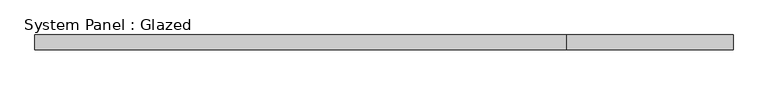
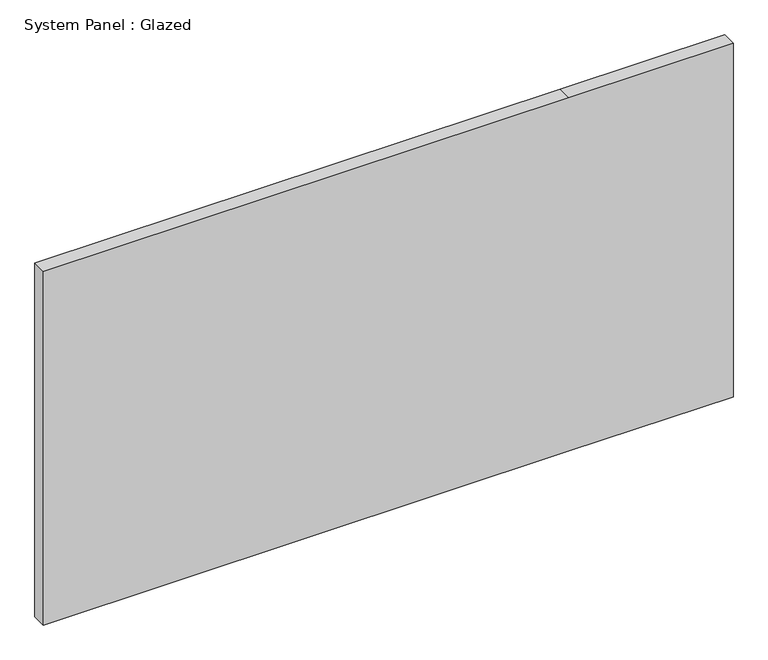
"""IFC4 building model written with IfcOpenShell, lengths in millimetres: plate geometry, System Panel : Glazed."""

import ifcopenshell
import ifcopenshell.guid

model = None  # the IFC model being written
_history = None  # IfcOwnerHistory: only IFC2X3 demands one
_inside = {}  # id of a spatial element -> (the spatial element, [elements in it])
_under = {}  # id of a project, library or spatial element -> (it, [spatial elements below it])
_declared = {}  # id of a project -> (the project, [libraries it declares])
_typed = {}  # id of a type object -> (the type object, [elements of that type])
_made_of = {}  # id of a material, layer set ... -> (it, [elements and type objects made of it])


def new_model(schema):
    """Start an empty IFC model of exactly this schema.

    Asked for "IFC4X3", IfcOpenShell would pick the latest addendum, in which some entities
    have other attributes; the version numbers below select the first issue.
    IFC2X3 requires an IfcOwnerHistory on every rooted entity: one is made here for all.
    """
    global model, _history
    if schema == "IFC4X3":
        model = ifcopenshell.file(schema_version=(4, 3, 0, 0))
    else:
        model = ifcopenshell.file(schema=schema)
    _inside.clear()
    _under.clear()
    _declared.clear()
    _typed.clear()
    _made_of.clear()
    _history = None
    if model.schema == "IFC2X3":
        org = make("IfcOrganization", Name="unknown")
        user = make(
            "IfcPersonAndOrganization",
            ThePerson=make("IfcPerson", FamilyName="unknown"),
            TheOrganization=org,
        )
        app = make(
            "IfcApplication",
            ApplicationDeveloper=org,
            Version="unknown",
            ApplicationFullName="unknown",
            ApplicationIdentifier="unknown",
        )
        _history = make(
            "IfcOwnerHistory",
            OwningUser=user,
            OwningApplication=app,
            ChangeAction="ADDED",
            CreationDate=0,
        )
    return model


def make(cls, **values):
    """One entity of the class cls with the attributes given. An attribute that is None is left unset."""
    return model.create_entity(
        cls, **{name: value for name, value in values.items() if value is not None}
    )


def rooted(cls, **values):
    """An entity with a GlobalId (a new one), such as an element, a storey or a relation."""
    return make(cls, GlobalId=ifcopenshell.guid.new(), OwnerHistory=_history, **values)


def si_unit(unit_type, name, prefix=None):
    """IfcSIUnit, for example si_unit("LENGTHUNIT", "METRE", prefix="MILLI")."""
    return make("IfcSIUnit", UnitType=unit_type, Prefix=prefix, Name=name)


def assignment(units):
    """IfcUnitAssignment: the units of a project."""
    return None if units is None else make("IfcUnitAssignment", Units=units)


def point(xyz):
    """IfcCartesianPoint."""
    return None if xyz is None else make("IfcCartesianPoint", Coordinates=xyz)


def direction(xyz):
    """IfcDirection."""
    return None if xyz is None else make("IfcDirection", DirectionRatios=xyz)


def frame(location, z_axis=None, x_axis=None):
    """IfcAxis2Placement3D, a coordinate frame: its origin and axes. An axis left out is left unset."""
    return make(
        "IfcAxis2Placement3D",
        Location=point(location),
        Axis=direction(z_axis),
        RefDirection=direction(x_axis),
    )


def origin():
    """The frame at (0, 0, 0) with its axes left unset."""
    return frame((0.0, 0.0, 0.0))


def place(relative_to, where):
    """IfcLocalPlacement: puts the frame where relative to a parent placement (None: the world)."""
    return make(
        "IfcLocalPlacement", PlacementRelTo=relative_to, RelativePlacement=where
    )


def context(
    kind, dimensions, precision=None, world=None, true_north=None, identifier=None
):
    """IfcGeometricRepresentationContext, for example the 3D "Model" context."""
    return make(
        "IfcGeometricRepresentationContext",
        ContextIdentifier=identifier,
        ContextType=kind,
        CoordinateSpaceDimension=dimensions,
        Precision=precision,
        WorldCoordinateSystem=world,
        TrueNorth=true_north,
    )


def project(units=None, contexts=None):
    """IfcProject with its units and contexts."""
    return rooted(
        "IfcProject",
        Name="project",
        RepresentationContexts=contexts,
        UnitsInContext=assignment(units),
    )


def spatial(cls, under=None, at=None, **own):
    """A site, building, storey or space (cls), placed at a placement, below another one or the project."""
    s = rooted(cls, ObjectPlacement=at, **own)
    if under is not None:
        _under.setdefault(under.id(), (under, []))[1].append(s)
    return s


def polyline(points):
    """IfcPolyline through the points."""
    return make("IfcPolyline", Points=[point(p) for p in points])


def outline(outer, holes=None, kind="AREA"):
    """IfcArbitraryClosedProfileDef: a profile drawn as a closed curve; with holes, ...WithVoids."""
    if holes is None:
        return make("IfcArbitraryClosedProfileDef", ProfileType=kind, OuterCurve=outer)
    return make(
        "IfcArbitraryProfileDefWithVoids",
        ProfileType=kind,
        OuterCurve=outer,
        InnerCurves=holes,
    )


def extrude(swept, where, along, depth):
    """IfcExtrudedAreaSolid: the profile swept, set in the frame where, extruded along a direction by depth."""
    return make(
        "IfcExtrudedAreaSolid",
        SweptArea=swept,
        Position=where,
        ExtrudedDirection=direction(along),
        Depth=depth,
    )


def shape(context_of_items, identifier, shape_type, items):
    """IfcShapeRepresentation: the items that make up one representation, for example the "Body"."""
    return make(
        "IfcShapeRepresentation",
        ContextOfItems=context_of_items,
        RepresentationIdentifier=identifier,
        RepresentationType=shape_type,
        Items=items,
    )


def source(mapping_origin, context_of_items, identifier, shape_type, items):
    """IfcRepresentationMap: a shape defined once, which mapped items show again and again."""
    return make(
        "IfcRepresentationMap",
        MappingOrigin=mapping_origin,
        MappedRepresentation=shape(context_of_items, identifier, shape_type, items),
    )


def transform(
    local_origin,
    x_axis=None,
    y_axis=None,
    z_axis=None,
    scale=None,
    scale2=None,
    scale3=None,
    uniform=True,
):
    """IfcCartesianTransformationOperator3D, or its non-uniform kind. x_axis, y_axis, z_axis: its Axis1, 2, 3."""
    if uniform:
        return make(
            "IfcCartesianTransformationOperator3D",
            Axis1=direction(x_axis),
            Axis2=direction(y_axis),
            LocalOrigin=point(local_origin),
            Scale=scale,
            Axis3=direction(z_axis),
        )
    return make(
        "IfcCartesianTransformationOperator3DnonUniform",
        Axis1=direction(x_axis),
        Axis2=direction(y_axis),
        LocalOrigin=point(local_origin),
        Scale=scale,
        Axis3=direction(z_axis),
        Scale2=scale2,
        Scale3=scale3,
    )


def mapped(mapping_source, mapping_target):
    """IfcMappedItem: shows the shape of a source again, moved by a transform."""
    return make(
        "IfcMappedItem", MappingSource=mapping_source, MappingTarget=mapping_target
    )


def made_of(thing, what):
    """Note that an element or type object is made of a material, layer set ...; save() writes the relation."""
    if what is not None:
        _made_of.setdefault(what.id(), (what, []))[1].append(thing)
    return thing


def element(
    cls,
    number,
    at=None,
    inside=None,
    cuts=None,
    type_object=None,
    material=None,
    context=None,
    identifier="Body",
    shape_type=None,
    held_by="IfcProductDefinitionShape",
    body=None,
    shapes=None,
    **own,
):
    """One element of the class cls, such as IfcWall. Its Tag is "e" and its number.

    at: its placement. inside: the storey or other place that contains it. cuts: it is an
    opening in that element (IfcRelVoidsElement). A single representation is given by context,
    identifier, shape_type and body (its items); several are given by shapes. held_by: the class
    of the entity that holds the representations. save() writes the other relations.
    """
    e = rooted(cls, Tag="e%d" % number, ObjectPlacement=at, **own)
    if body is not None:
        shapes = [shape(context, identifier, shape_type, body)]
    if shapes is not None:
        e.Representation = make(held_by, Representations=shapes)
    if inside is not None:
        _inside.setdefault(inside.id(), (inside, []))[1].append(e)
    if cuts is not None:
        rooted(
            "IfcRelVoidsElement", RelatingBuildingElement=cuts, RelatedOpeningElement=e
        )
    if type_object is not None:
        _typed.setdefault(type_object.id(), (type_object, []))[1].append(e)
    return made_of(e, material)


def aggregate(whole, parts):
    """IfcRelAggregates: a whole, such as a stair, and the parts it consists of."""
    return rooted("IfcRelAggregates", RelatingObject=whole, RelatedObjects=parts)


def save(model, path):
    """Write the relations noted so far, then the file.

    IfcRelAggregates (storeys below a building ...), IfcRelContainedInSpatialStructure (elements
    in a storey), IfcRelDefinesByType, IfcRelAssociatesMaterial and IfcRelDeclares: one each for
    every whole, place, type object, material and project.
    """
    for whole, parts in _under.values():
        aggregate(whole, parts)
    for where, things in _inside.values():
        rooted(
            "IfcRelContainedInSpatialStructure",
            RelatedElements=things,
            RelatingStructure=where,
        )
    for kind, things in _typed.values():
        rooted("IfcRelDefinesByType", RelatedObjects=things, RelatingType=kind)
    for what, things in _made_of.values():
        rooted("IfcRelAssociatesMaterial", RelatedObjects=things, RelatingMaterial=what)
    for by, libraries in _declared.values():
        rooted("IfcRelDeclares", RelatingContext=by, RelatedDefinitions=libraries)
    model.write(path)


def system_panel_glazed_128d3776(model_context):
    return source(origin(), model_context, "Body", "SweptSolid", [
        extrude(outline(polyline([(0.0, -600.075), (0.0, 314.325), (0.0, 600.075), (650.875, 600.075), (650.875, 314.325), (650.875, -600.075), (0.0, -600.075)])), frame((0.0, -44.45, 0.0), z_axis=(0.0, 1.0, 0.0), x_axis=(0.0, 0.0, 1.0)), (0.0, 0.0, 1.0), 25.4),
    ])


if __name__ == "__main__":
    model = new_model("IFC4")
    model_context = context("Model", 3, world=origin())
    ifc_project = project(units=[si_unit("LENGTHUNIT", "METRE", prefix="MILLI")], contexts=[model_context])
    site = spatial("IfcSite", under=ifc_project)
    building = spatial("IfcBuilding", under=site)
    placement = place(None, origin())
    system_panel_glazed_shape = system_panel_glazed_128d3776(model_context)
    element("IfcPlate", 1, ObjectType="System Panel : Glazed", at=placement, inside=building, context=model_context, shape_type="MappedRepresentation", body=[
        mapped(system_panel_glazed_shape, transform((0.0, 0.0, 0.0), x_axis=(1.0, 0.0, 0.0), y_axis=(0.0, 1.0, 0.0), z_axis=(0.0, 0.0, 1.0))),
    ])
    save(model, "model.ifc")

# Revit data of these elements
# Type "System Panel : Glazed"
#   Construction Type Id = "GSP4R"
#   Analytic Construction = "1/8 in Pilkington single glazing"
#   Visual Light Transmittance = 0.9
#   Solar Heat Gain Coefficient = 0.86
#   Heat Transfer Coefficient (U) = 1.18115 BTU/(h·ft²·°F)
#   Define Thermal Properties by = 1
# Element 1 (IfcPlate, "System Panel : Glazed")
#   Materials on its faces: "Glass"
# Materials
#   "Glass": class "Glass", colour RGB 0 128 192, transparency 0.75, Description = "Soda Lime Glass", Cost = 0
